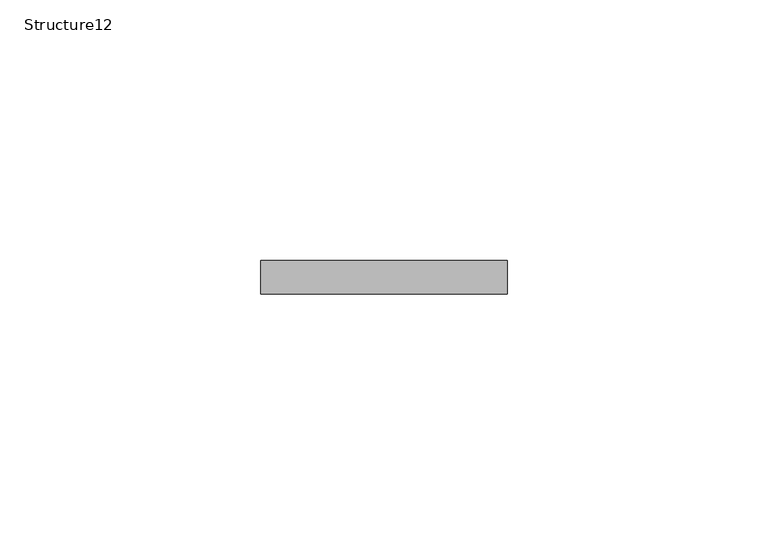
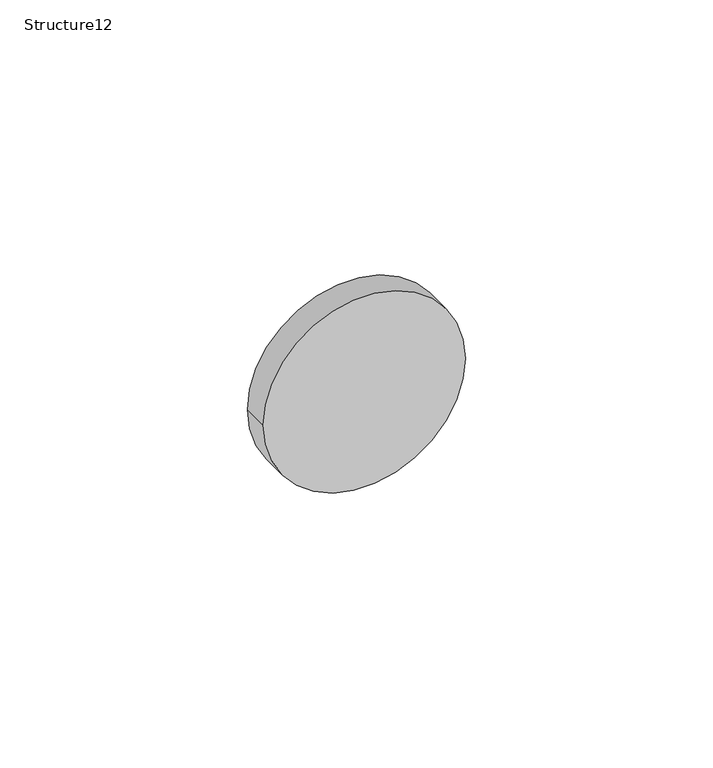
"""IFC4 building model written with IfcOpenShell, lengths in millimetres: proxy geometry, Structure12 : Structure668217133."""

from ifc_helpers import new_model, si_unit, point, frame, frame_2d, origin, place, context, project, spatial, circle_curve, trimmed, segment, composite_curve, outline, extrude, source, transform, mapped, element, save


def structure12_e36a5ae5(model_context):
    return source(origin(), model_context, "Body", "SweptSolid", [
        extrude(outline(composite_curve([segment(trimmed(circle_curve(frame_2d((38047.8454063, 5185.7383658)), 23.5716554), [point((38047.8454063, 5162.1667104))], [point((38047.8454063, 5209.3100213))], False, "CARTESIAN"), True, "CONTINUOUS"), segment(trimmed(circle_curve(frame_2d((38047.8454063, 5185.7383658)), 23.5716554), [point((38047.8454063, 5209.3100213))], [point((38047.8454063, 5162.1667104))], False, "CARTESIAN"), True, "CONTINUOUS")], self_intersect=False)), frame((0.0, 1957.9072934, 0.0), z_axis=(0.0, 1.0, 0.0), x_axis=(0.0, 0.0, 1.0)), (0.0, 0.0, 1.0), 6.35),
    ])


if __name__ == "__main__":
    model = new_model("IFC4")
    model_context = context("Model", 3, world=origin())
    ifc_project = project(units=[si_unit("LENGTHUNIT", "METRE", prefix="MILLI")], contexts=[model_context])
    site = spatial("IfcSite", under=ifc_project)
    building = spatial("IfcBuilding", under=site)
    placement = place(None, origin())
    structure12_shape = structure12_e36a5ae5(model_context)
    element("IfcBuildingElementProxy", 1, Name="Structure12 : Structure668217133", ObjectType="Structure12 : Structure668217133", at=placement, inside=building, context=model_context, shape_type="MappedRepresentation", body=[
        mapped(structure12_shape, transform((0.0, 0.0, 0.0), x_axis=(1.0, 0.0, 0.0), y_axis=(0.0, 1.0, 0.0), z_axis=(0.0, 0.0, 1.0))),
    ])
    save(model, "model.ifc")

# Revit data of these elements
# Type "Structure12 : Structure668217133"
#   NameOverride = "Structure668217133"
# Element 1 (IfcBuildingElementProxy, "Structure12 : Structure668217133")
#   Materials on its faces: "RUBBER GASKET"
# Materials
#   "RUBBER GASKET": class "Unassigned", colour RGB 70 70 70, transparency 0
